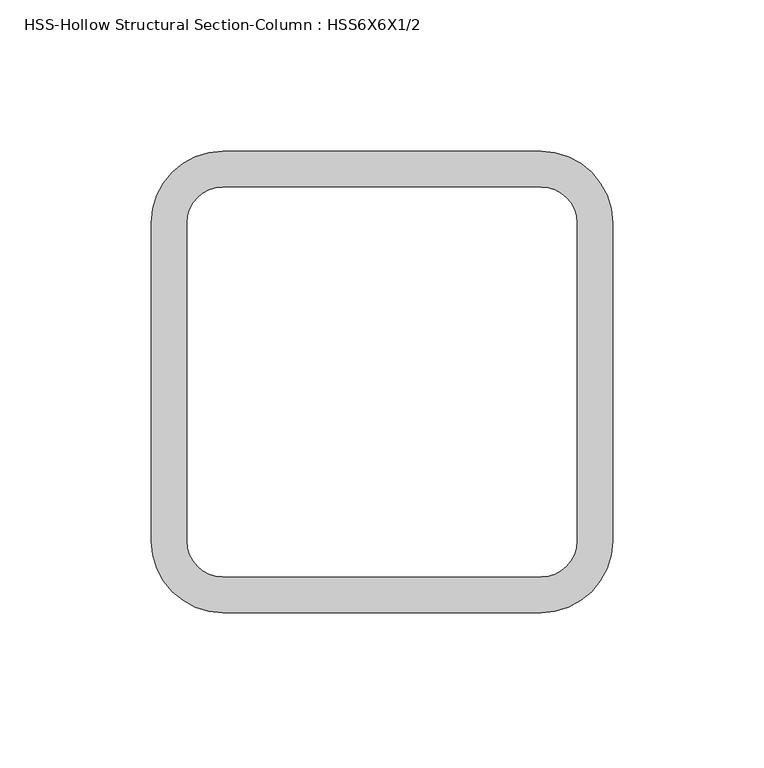
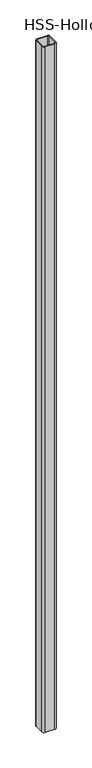
"""IFC4 building model written with IfcOpenShell, lengths in millimetres: column geometry, HSS-Hollow Structural Section-Column : HSS6X6X1/2."""

from ifc_helpers import new_model, si_unit, point, frame, frame_2d, origin, place, context, project, spatial, polyline, circle_curve, trimmed, segment, composite_curve, outline, extrude, source, transform, mapped, element, save


def hss_hollow_structural_section_column_hss6x6x1_2_896db910(model_context):
    return source(origin(), model_context, "Body", "SweptSolid", [
        extrude(outline(composite_curve([segment(trimmed(circle_curve(frame_2d((52.578, 52.578)), 23.622), [point((52.578, 76.2))], [point((76.2, 52.578))], False, "CARTESIAN"), True, "CONTINUOUS"), segment(polyline([(76.2, 52.578), (76.2, -52.578)]), True, "CONTINUOUS"), segment(trimmed(circle_curve(frame_2d((52.578, -52.578)), 23.622), [point((76.2, -52.578))], [point((52.578, -76.2))], False, "CARTESIAN"), True, "CONTINUOUS"), segment(polyline([(52.578, -76.2), (-52.578, -76.2)]), True, "CONTINUOUS"), segment(trimmed(circle_curve(frame_2d((-52.578, -52.578)), 23.622), [point((-52.578, -76.2))], [point((-76.2, -52.578))], False, "CARTESIAN"), True, "CONTINUOUS"), segment(polyline([(-76.2, -52.578), (-76.2, 52.578)]), True, "CONTINUOUS"), segment(trimmed(circle_curve(frame_2d((-52.578, 52.578)), 23.622), [point((-76.2, 52.578))], [point((-52.578, 76.2))], False, "CARTESIAN"), True, "CONTINUOUS"), segment(polyline([(-52.578, 76.2), (52.578, 76.2)]), True, "CONTINUOUS")], self_intersect=False), holes=[composite_curve([segment(polyline([(52.578, 64.389), (-52.578, 64.389)]), True, "CONTINUOUS"), segment(trimmed(circle_curve(frame_2d((-52.578, 52.578)), 11.811), [point((-52.578, 64.389))], [point((-64.389, 52.578))], True, "CARTESIAN"), True, "CONTINUOUS"), segment(polyline([(-64.389, 52.578), (-64.389, -52.578)]), True, "CONTINUOUS"), segment(trimmed(circle_curve(frame_2d((-52.578, -52.578)), 11.811), [point((-64.389, -52.578))], [point((-52.578, -64.389))], True, "CARTESIAN"), True, "CONTINUOUS"), segment(polyline([(-52.578, -64.389), (52.578, -64.389)]), True, "CONTINUOUS"), segment(trimmed(circle_curve(frame_2d((52.578, -52.578)), 11.811), [point((52.578, -64.389))], [point((64.389, -52.578))], True, "CARTESIAN"), True, "CONTINUOUS"), segment(polyline([(64.389, -52.578), (64.389, 52.578)]), True, "CONTINUOUS"), segment(trimmed(circle_curve(frame_2d((52.578, 52.578)), 11.811), [point((64.389, 52.578))], [point((52.578, 64.389))], True, "CARTESIAN"), True, "CONTINUOUS")], self_intersect=False)]), frame((0.0, 0.0, 4267.2), z_axis=(0.0, 0.0, 1.0), x_axis=(1.0, 0.0, 0.0)), (0.0, 0.0, 1.0), 7899.4),
    ])


if __name__ == "__main__":
    model = new_model("IFC4")
    model_context = context("Model", 3, world=origin())
    ifc_project = project(units=[si_unit("LENGTHUNIT", "METRE", prefix="MILLI")], contexts=[model_context])
    site = spatial("IfcSite", under=ifc_project)
    building = spatial("IfcBuilding", under=site)
    placement = place(None, origin())
    hss_hollow_structural_section_column_hss6x6x1_2_shape = hss_hollow_structural_section_column_hss6x6x1_2_896db910(model_context)
    element("IfcColumn", 1, ObjectType="HSS-Hollow Structural Section-Column : HSS6X6X1/2", at=placement, inside=building, context=model_context, shape_type="MappedRepresentation", body=[
        mapped(hss_hollow_structural_section_column_hss6x6x1_2_shape, transform((0.0, 0.0, 0.0), x_axis=(1.0, 0.0, 0.0), y_axis=(0.0, 1.0, 0.0), z_axis=(0.0, 0.0, 1.0))),
    ])
    save(model, "model.ifc")

# Revit data of these elements
# Type "HSS-Hollow Structural Section-Column : HSS6X6X1/2"
#   Assembly Code = "B10"
#   Shape = "Square"
#   W = 35.1
#   Ht = 0' - 6"
#   b = 0' - 6"
#   kr = 0' - 0.93"
#   t = 0' - 0.465"
#   A = 0.0676389 SF
#   Structural Material [instance default] = Steel ASTM A500, Grade B, Rectangular and Square
# Element 1 (IfcColumn, "HSS-Hollow Structural Section-Column : HSS6X6X1/2")
#   Materials on its faces: "Steel ASTM A500, Grade B, Rectangular and Square"
# Materials
#   "Steel ASTM A500, Grade B, Rectangular and Square": class "Metal", colour RGB 199 199 199, transparency 0, Description = "Carbon steel", Cost = 0
